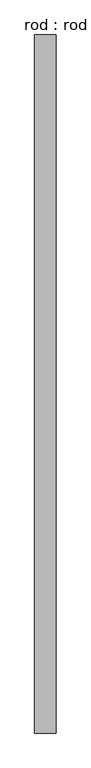
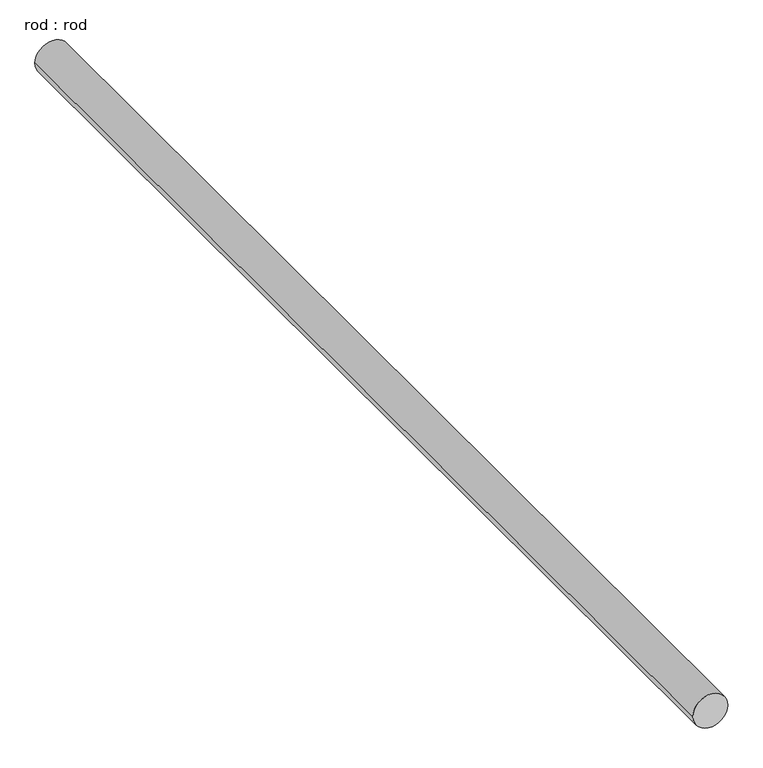
"""IFC4 building model written with IfcOpenShell, lengths in millimetres: proxy geometry, rod : rod."""

from ifc_helpers import new_model, si_unit, point, frame, frame_2d, origin, place, context, project, spatial, circle_curve, trimmed, segment, composite_curve, outline, extrude, source, transform, mapped, element, save


def rod_rod_b823eda0(model_context):
    return source(origin(), model_context, "Body", "SweptSolid", [
        extrude(outline(composite_curve([segment(trimmed(circle_curve(frame_2d((0.0108462, 0.0)), 200.0), [point((0.0108462, 200.0))], [point((0.0108462, -200.0))], False, "CARTESIAN"), True, "CONTINUOUS"), segment(trimmed(circle_curve(frame_2d((0.0108462, 0.0)), 200.0), [point((0.0108462, -200.0))], [point((0.0108462, 200.0))], False, "CARTESIAN"), True, "CONTINUOUS")], self_intersect=False)), frame((0.0, -2435.0491624, 0.0), z_axis=(0.0, 1.0, 0.0), x_axis=(0.0, 0.0, 1.0)), (0.0, 0.0, 1.0), 13055.5555556),
    ])


if __name__ == "__main__":
    model = new_model("IFC4")
    model_context = context("Model", 3, world=origin())
    ifc_project = project(units=[si_unit("LENGTHUNIT", "METRE", prefix="MILLI")], contexts=[model_context])
    site = spatial("IfcSite", under=ifc_project)
    building = spatial("IfcBuilding", under=site)
    placement = place(None, origin())
    rod_rod_shape = rod_rod_b823eda0(model_context)
    element("IfcBuildingElementProxy", 1, Name="rod : rod", ObjectType="rod : rod", at=placement, inside=building, context=model_context, shape_type="MappedRepresentation", body=[
        mapped(rod_rod_shape, transform((0.0, 0.0, 0.0), x_axis=(1.0, 0.0, 0.0), y_axis=(0.0, 1.0, 0.0), z_axis=(0.0, 0.0, 1.0))),
    ])
    save(model, "model.ifc")

# Revit data of these elements
# Type "rod : rod"
#   Default Elevation = 0
